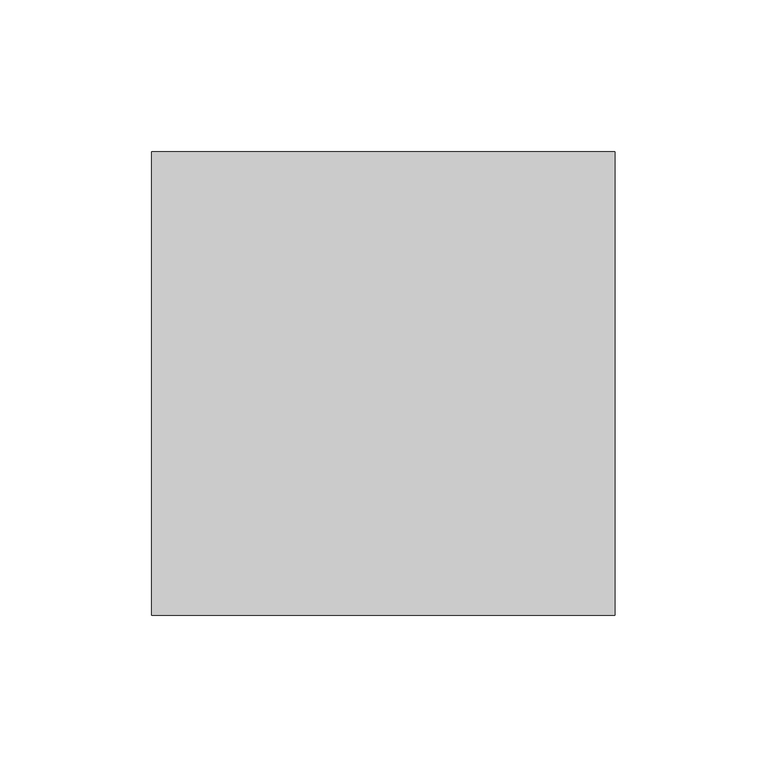
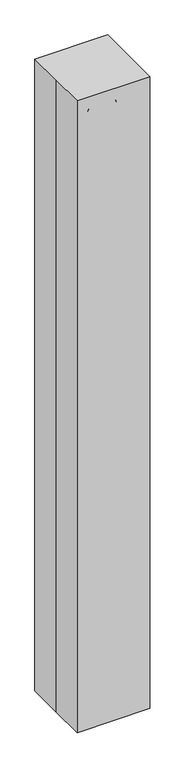
"""IFC4 building model written with IfcOpenShell, lengths in millimetres: proxy geometry, M8515 - Gastroscope, Fiberoptic, Therapeutic : M8515 - Gastroscope, Fiberoptic, Therapeutic."""

import ifcopenshell
import ifcopenshell.guid

model = None  # the IFC model being written
_history = None  # IfcOwnerHistory: only IFC2X3 demands one
_inside = {}  # id of a spatial element -> (the spatial element, [elements in it])
_under = {}  # id of a project, library or spatial element -> (it, [spatial elements below it])
_declared = {}  # id of a project -> (the project, [libraries it declares])
_typed = {}  # id of a type object -> (the type object, [elements of that type])
_made_of = {}  # id of a material, layer set ... -> (it, [elements and type objects made of it])


def new_model(schema):
    """Start an empty IFC model of exactly this schema.

    Asked for "IFC4X3", IfcOpenShell would pick the latest addendum, in which some entities
    have other attributes; the version numbers below select the first issue.
    IFC2X3 requires an IfcOwnerHistory on every rooted entity: one is made here for all.
    """
    global model, _history
    if schema == "IFC4X3":
        model = ifcopenshell.file(schema_version=(4, 3, 0, 0))
    else:
        model = ifcopenshell.file(schema=schema)
    _inside.clear()
    _under.clear()
    _declared.clear()
    _typed.clear()
    _made_of.clear()
    _history = None
    if model.schema == "IFC2X3":
        org = make("IfcOrganization", Name="unknown")
        user = make(
            "IfcPersonAndOrganization",
            ThePerson=make("IfcPerson", FamilyName="unknown"),
            TheOrganization=org,
        )
        app = make(
            "IfcApplication",
            ApplicationDeveloper=org,
            Version="unknown",
            ApplicationFullName="unknown",
            ApplicationIdentifier="unknown",
        )
        _history = make(
            "IfcOwnerHistory",
            OwningUser=user,
            OwningApplication=app,
            ChangeAction="ADDED",
            CreationDate=0,
        )
    return model


def make(cls, **values):
    """One entity of the class cls with the attributes given. An attribute that is None is left unset."""
    return model.create_entity(
        cls, **{name: value for name, value in values.items() if value is not None}
    )


def rooted(cls, **values):
    """An entity with a GlobalId (a new one), such as an element, a storey or a relation."""
    return make(cls, GlobalId=ifcopenshell.guid.new(), OwnerHistory=_history, **values)


def si_unit(unit_type, name, prefix=None):
    """IfcSIUnit, for example si_unit("LENGTHUNIT", "METRE", prefix="MILLI")."""
    return make("IfcSIUnit", UnitType=unit_type, Prefix=prefix, Name=name)


def assignment(units):
    """IfcUnitAssignment: the units of a project."""
    return None if units is None else make("IfcUnitAssignment", Units=units)


def point(xyz):
    """IfcCartesianPoint."""
    return None if xyz is None else make("IfcCartesianPoint", Coordinates=xyz)


def direction(xyz):
    """IfcDirection."""
    return None if xyz is None else make("IfcDirection", DirectionRatios=xyz)


def frame(location, z_axis=None, x_axis=None):
    """IfcAxis2Placement3D, a coordinate frame: its origin and axes. An axis left out is left unset."""
    return make(
        "IfcAxis2Placement3D",
        Location=point(location),
        Axis=direction(z_axis),
        RefDirection=direction(x_axis),
    )


def origin():
    """The frame at (0, 0, 0) with its axes left unset."""
    return frame((0.0, 0.0, 0.0))


def origin_with_axes():
    """The frame at (0, 0, 0) with the z axis (0, 0, 1) and the x axis (1, 0, 0) written out."""
    return frame((0.0, 0.0, 0.0), z_axis=(0.0, 0.0, 1.0), x_axis=(1.0, 0.0, 0.0))


def place(relative_to, where):
    """IfcLocalPlacement: puts the frame where relative to a parent placement (None: the world)."""
    return make(
        "IfcLocalPlacement", PlacementRelTo=relative_to, RelativePlacement=where
    )


def context(
    kind, dimensions, precision=None, world=None, true_north=None, identifier=None
):
    """IfcGeometricRepresentationContext, for example the 3D "Model" context."""
    return make(
        "IfcGeometricRepresentationContext",
        ContextIdentifier=identifier,
        ContextType=kind,
        CoordinateSpaceDimension=dimensions,
        Precision=precision,
        WorldCoordinateSystem=world,
        TrueNorth=true_north,
    )


def project(units=None, contexts=None):
    """IfcProject with its units and contexts."""
    return rooted(
        "IfcProject",
        Name="project",
        RepresentationContexts=contexts,
        UnitsInContext=assignment(units),
    )


def spatial(cls, under=None, at=None, **own):
    """A site, building, storey or space (cls), placed at a placement, below another one or the project."""
    s = rooted(cls, ObjectPlacement=at, **own)
    if under is not None:
        _under.setdefault(under.id(), (under, []))[1].append(s)
    return s


def polyline(points):
    """IfcPolyline through the points."""
    return make("IfcPolyline", Points=[point(p) for p in points])


def circle_curve(where, radius):
    """IfcCircle in the frame where."""
    return make("IfcCircle", Position=where, Radius=radius)


def ellipse_curve(where, semi_axis1, semi_axis2):
    """IfcEllipse in the frame where."""
    return make(
        "IfcEllipse", Position=where, SemiAxis1=semi_axis1, SemiAxis2=semi_axis2
    )


def trimmed(basis, trim1, trim2, sense, master):
    """IfcTrimmedCurve: the piece of a basis curve between two trims."""
    return make(
        "IfcTrimmedCurve",
        BasisCurve=basis,
        Trim1=trim1,
        Trim2=trim2,
        SenseAgreement=sense,
        MasterRepresentation=master,
    )


def outline(outer, holes=None, kind="AREA"):
    """IfcArbitraryClosedProfileDef: a profile drawn as a closed curve; with holes, ...WithVoids."""
    if holes is None:
        return make("IfcArbitraryClosedProfileDef", ProfileType=kind, OuterCurve=outer)
    return make(
        "IfcArbitraryProfileDefWithVoids",
        ProfileType=kind,
        OuterCurve=outer,
        InnerCurves=holes,
    )


def extrude(swept, where, along, depth):
    """IfcExtrudedAreaSolid: the profile swept, set in the frame where, extruded along a direction by depth."""
    return make(
        "IfcExtrudedAreaSolid",
        SweptArea=swept,
        Position=where,
        ExtrudedDirection=direction(along),
        Depth=depth,
    )


def shape(context_of_items, identifier, shape_type, items):
    """IfcShapeRepresentation: the items that make up one representation, for example the "Body"."""
    return make(
        "IfcShapeRepresentation",
        ContextOfItems=context_of_items,
        RepresentationIdentifier=identifier,
        RepresentationType=shape_type,
        Items=items,
    )


def source(mapping_origin, context_of_items, identifier, shape_type, items):
    """IfcRepresentationMap: a shape defined once, which mapped items show again and again."""
    return make(
        "IfcRepresentationMap",
        MappingOrigin=mapping_origin,
        MappedRepresentation=shape(context_of_items, identifier, shape_type, items),
    )


def transform(
    local_origin,
    x_axis=None,
    y_axis=None,
    z_axis=None,
    scale=None,
    scale2=None,
    scale3=None,
    uniform=True,
):
    """IfcCartesianTransformationOperator3D, or its non-uniform kind. x_axis, y_axis, z_axis: its Axis1, 2, 3."""
    if uniform:
        return make(
            "IfcCartesianTransformationOperator3D",
            Axis1=direction(x_axis),
            Axis2=direction(y_axis),
            LocalOrigin=point(local_origin),
            Scale=scale,
            Axis3=direction(z_axis),
        )
    return make(
        "IfcCartesianTransformationOperator3DnonUniform",
        Axis1=direction(x_axis),
        Axis2=direction(y_axis),
        LocalOrigin=point(local_origin),
        Scale=scale,
        Axis3=direction(z_axis),
        Scale2=scale2,
        Scale3=scale3,
    )


def mapped(mapping_source, mapping_target):
    """IfcMappedItem: shows the shape of a source again, moved by a transform."""
    return make(
        "IfcMappedItem", MappingSource=mapping_source, MappingTarget=mapping_target
    )


def made_of(thing, what):
    """Note that an element or type object is made of a material, layer set ...; save() writes the relation."""
    if what is not None:
        _made_of.setdefault(what.id(), (what, []))[1].append(thing)
    return thing


def element(
    cls,
    number,
    at=None,
    inside=None,
    cuts=None,
    type_object=None,
    material=None,
    context=None,
    identifier="Body",
    shape_type=None,
    held_by="IfcProductDefinitionShape",
    body=None,
    shapes=None,
    **own,
):
    """One element of the class cls, such as IfcWall. Its Tag is "e" and its number.

    at: its placement. inside: the storey or other place that contains it. cuts: it is an
    opening in that element (IfcRelVoidsElement). A single representation is given by context,
    identifier, shape_type and body (its items); several are given by shapes. held_by: the class
    of the entity that holds the representations. save() writes the other relations.
    """
    e = rooted(cls, Tag="e%d" % number, ObjectPlacement=at, **own)
    if body is not None:
        shapes = [shape(context, identifier, shape_type, body)]
    if shapes is not None:
        e.Representation = make(held_by, Representations=shapes)
    if inside is not None:
        _inside.setdefault(inside.id(), (inside, []))[1].append(e)
    if cuts is not None:
        rooted(
            "IfcRelVoidsElement", RelatingBuildingElement=cuts, RelatedOpeningElement=e
        )
    if type_object is not None:
        _typed.setdefault(type_object.id(), (type_object, []))[1].append(e)
    return made_of(e, material)


def aggregate(whole, parts):
    """IfcRelAggregates: a whole, such as a stair, and the parts it consists of."""
    return rooted("IfcRelAggregates", RelatingObject=whole, RelatedObjects=parts)


def save(model, path):
    """Write the relations noted so far, then the file.

    IfcRelAggregates (storeys below a building ...), IfcRelContainedInSpatialStructure (elements
    in a storey), IfcRelDefinesByType, IfcRelAssociatesMaterial and IfcRelDeclares: one each for
    every whole, place, type object, material and project.
    """
    for whole, parts in _under.values():
        aggregate(whole, parts)
    for where, things in _inside.values():
        rooted(
            "IfcRelContainedInSpatialStructure",
            RelatedElements=things,
            RelatingStructure=where,
        )
    for kind, things in _typed.values():
        rooted("IfcRelDefinesByType", RelatedObjects=things, RelatingType=kind)
    for what, things in _made_of.values():
        rooted("IfcRelAssociatesMaterial", RelatedObjects=things, RelatingMaterial=what)
    for by, libraries in _declared.values():
        rooted("IfcRelDeclares", RelatingContext=by, RelatedDefinitions=libraries)
    model.write(path)


def plane_surface(at):
    """IfcPlane: the flat surface through the origin of the frame at, square to its z axis."""
    return make("IfcPlane", Position=at)


def cylinder_surface(at, radius):
    """IfcCylindricalSurface: all points at the distance radius from the z axis of the frame at."""
    return make("IfcCylindricalSurface", Position=at, Radius=radius)


def revolved_surface(curve, axis_point, axis_direction):
    """IfcSurfaceOfRevolution: the curve turned about the line through axis_point along axis_direction."""
    return make(
        "IfcSurfaceOfRevolution",
        SweptCurve=make("IfcArbitraryOpenProfileDef", ProfileType="CURVE", Curve=curve),
        AxisPosition=make("IfcAxis1Placement", Location=point(axis_point), Axis=direction(axis_direction)),
    )


def advanced_brep(points, edges, surfaces, faces):
    """IfcAdvancedBrep: a solid bounded by faces that lie on surfaces and meet in shared edges.

    An edge is (start, end): straight between two places in points (the first is 0);
    or (start, end, curve); or (start, end, curve, False) where it runs against its curve.
    A face is (place in surfaces, loops), or (place, loops, False) where it looks against
    its surface's normal. A loop lists edges by number (the first is 1), with a minus sign
    where the edge is run from its end to its start. The first loop is the outer one.
    """
    corners = [point(p) for p in points]
    vertices = [make("IfcVertexPoint", VertexGeometry=c) for c in corners]
    made = []
    for start, end, *more in edges:
        made.append(
            make(
                "IfcEdgeCurve",
                EdgeStart=vertices[start],
                EdgeEnd=vertices[end],
                EdgeGeometry=more[0] if more else make("IfcPolyline", Points=[corners[start], corners[end]]),
                SameSense=more[1] if len(more) > 1 else True,
            )
        )
    hull = []
    for where, loops, *sense in faces:
        bounds = []
        for j, loop in enumerate(loops):
            ring = [make("IfcOrientedEdge", EdgeElement=made[abs(k) - 1], Orientation=k > 0) for k in loop]
            bounds.append(
                make(
                    "IfcFaceOuterBound" if j == 0 else "IfcFaceBound",
                    Bound=make("IfcEdgeLoop", EdgeList=ring),
                    Orientation=True,
                )
            )
        hull.append(make("IfcAdvancedFace", Bounds=bounds, FaceSurface=surfaces[where], SameSense=sense[0] if sense else True))
    return make("IfcAdvancedBrep", Outer=make("IfcClosedShell", CfsFaces=hull))


def specialty_equipment_7175bac1(model_context):
    return source(origin(), model_context, "Body", "SolidModel", [
        extrude(outline(polyline([(-12.7, -34.925), (-50.8, -34.925), (-50.8, -9.525), (-12.7, -9.525), (-12.7, -34.925)])), origin_with_axes(), (0.0, 0.0, 1.0), 101.6),
        advanced_brep(
        [(-25.4, -22.225, 101.6), (-38.1, -22.225, 101.6), (25.4, -22.225, 0.0), (38.1, -22.225, 0.0), (-25.4, -22.225, 1314.45), (-38.1, -22.225, 1314.45), (38.1, -22.225, 1314.45), (25.4, -22.225, 1314.45)],
        [
            (0, 1, circle_curve(frame((-31.75, -22.225, 101.6), z_axis=(0.0, 0.0, -1.0), x_axis=(-1.0, 0.0, 0.0)), 6.35)),
            (1, 0, circle_curve(frame((-31.75, -22.225, 101.6), z_axis=(0.0, 0.0, -1.0), x_axis=(-1.0, 0.0, 0.0)), 6.35)),
            (2, 3, circle_curve(frame((31.75, -22.225, 0.0), z_axis=(0.0, 0.0, -1.0), x_axis=(1.0, 0.0, 0.0)), 6.35)),
            (3, 2, circle_curve(frame((31.75, -22.225, 0.0), z_axis=(0.0, 0.0, -1.0), x_axis=(1.0, 0.0, 0.0)), 6.35)),
            (0, 4),
            (4, 5, circle_curve(frame((-31.75, -22.225, 1314.45), z_axis=(0.0, 0.0, -1.0), x_axis=(-1.0, 0.0, 0.0)), 6.35)),
            (5, 1),
            (5, 4, circle_curve(frame((-31.75, -22.225, 1314.45), z_axis=(0.0, 0.0, -1.0), x_axis=(-1.0, 0.0, 0.0)), 6.35)),
            (6, 7, circle_curve(frame((31.75, -22.225, 1314.45), z_axis=(0.0, 0.0, -1.0), x_axis=(1.0, 0.0, 0.0)), 6.35)),
            (7, 2),
            (3, 6),
            (7, 6, circle_curve(frame((31.75, -22.225, 1314.45), z_axis=(0.0, 0.0, -1.0), x_axis=(1.0, 0.0, 0.0)), 6.35)),
            (6, 5, circle_curve(frame((0.0, -22.225, 1314.45), z_axis=(0.0, -1.0, 0.0), x_axis=(-1.0, 0.0, 0.0)), 38.1)),
            (4, 7, circle_curve(frame((0.0, -22.225, 1314.45), z_axis=(0.0, 1.0, 0.0), x_axis=(-1.0, 0.0, 0.0)), 25.4)),
        ],
        [
            plane_surface(frame((-31.75, 41.275, 101.6), z_axis=(0.0, 0.0, -1.0), x_axis=(0.0, -1.0, 0.0))),
            plane_surface(frame((31.75, 41.275, 0.0), z_axis=(0.0, 0.0, -1.0), x_axis=(0.0, -1.0, 0.0))),
            cylinder_surface(frame((-31.75, -22.225, 101.6), z_axis=(0.0, 0.0, -1.0), x_axis=(-1.0, 0.0, 0.0)), 6.35),
            cylinder_surface(frame((31.75, -22.225, 1314.45), z_axis=(0.0, 0.0, 1.0), x_axis=(1.0, 0.0, 0.0)), 6.35),
            revolved_surface(trimmed(ellipse_curve(frame((-31.75, -22.225, 1314.45), z_axis=(0.0, 0.0, -1.0), x_axis=(-1.0, 0.0, 0.0)), 6.35, 6.35), [point((-25.4, -22.225, 1314.45))], [point((-38.1, -22.225, 1314.45))], True, "CARTESIAN"), (0.0, 41.275, 1314.45), (0.0, 1.0, 0.0)),
            revolved_surface(trimmed(ellipse_curve(frame((-31.75, -22.225, 1314.45), z_axis=(0.0, 0.0, -1.0), x_axis=(-1.0, 0.0, 0.0)), 6.35, 6.35), [point((-38.1, -22.225, 1314.45))], [point((-25.4, -22.225, 1314.45))], True, "CARTESIAN"), (0.0, 41.275, 1314.45), (0.0, 1.0, 0.0)),
        ],
        [
            (0, [[1, 2]]),
            (1, [[3, 4]]),
            (2, [[-1, 5, 6, 7]]),
            (2, [[-2, -7, 8, -5]]),
            (3, [[9, 10, -4, 11]]),
            (3, [[12, -11, -3, -10]]),
            (4, [[13, -6, 14, -9]]),
            (5, [[-14, -8, -13, -12]]),
        ],
    ),
        extrude(outline(polyline([(-76.2, 76.2), (76.2, 76.2), (76.2, -76.2), (-76.2, -76.2), (-76.2, 0.0), (-76.2, 76.2)])), origin_with_axes(), (0.0, 0.0, 1.0), 1397.0),
    ])


if __name__ == "__main__":
    model = new_model("IFC4")
    model_context = context("Model", 3, world=origin())
    ifc_project = project(units=[si_unit("LENGTHUNIT", "METRE", prefix="MILLI")], contexts=[model_context])
    site = spatial("IfcSite", under=ifc_project)
    building = spatial("IfcBuilding", under=site)
    placement = place(None, origin())
    specialty_equipment_shape = specialty_equipment_7175bac1(model_context)
    element("IfcBuildingElementProxy", 1, Name="M8515 - Gastroscope, Fiberoptic, Therapeutic : M8515 - Gastroscope, Fiberoptic, Therapeutic", ObjectType="M8515 - Gastroscope, Fiberoptic, Therapeutic : M8515 - Gastroscope, Fiberoptic, Therapeutic", at=placement, inside=building, context=model_context, shape_type="MappedRepresentation", body=[
        mapped(specialty_equipment_shape, transform((0.0, 0.0, 0.0), x_axis=(1.0, 0.0, 0.0), y_axis=(0.0, 1.0, 0.0), z_axis=(0.0, 0.0, 1.0))),
    ])
    save(model, "model.ifc")

# Revit data of these elements
# Type "M8515 - Gastroscope, Fiberoptic, Therapeutic : M8515 - Gastroscope, Fiberoptic, Therapeutic"
#   Watts2 = "0"
#   Watts1 = "0"
#   Unit_Issue = "EA"
#   UTIL_6_Misc = "-"
#   UTIL_5_NonMedGas = "-"
#   UTIL_4_MiscGas = "-"
#   UTIL_3_MedGas = "-"
#   UTIL_2_Elec = "-"
#   UTIL_1_WaterDrain = "-"
#   Nomenclature = "Gastroscope, Fiberoptic, Therapeutic"
#   NSN = "6515"
#   Location [instance default] = ""
#   JSN = "M8515"
#   Fund_Source_VA = "-"
#   Fund_Source_Navy = "-"
#   Fund_Source_Army = "-"
#   Fund_Source_AF = "-"
#   ELEC_Volts2 = "0"
#   ELEC_Volts1 = "0"
#   ELEC_Phase2 = "0"
#   ELEC_Phase1 = "0"
#   ELEC_HertzSwitch = "0"
#   ELEC_HertzDependent = "0"
#   ELEC_Hertz = "0"
#   ELEC_Amps2 = "0"
#   ELEC_Amps1 = "0"
#   DetailDescription = "Flexible fiberoptic gastroscope. This scope is designed for gastrointestinal exploration, cleaning, biopsy, tissue removal and suctioning. Unit consists of a thin flexible casing with a suction adapter, an instrument channel, light guides, an objective lens with an optical image fiber cluster, an air/water channel, an eyepiece and a cable for connection to a light source. Casings and instrument channels can have varying dimensions based on gastroscope design and intended procedure. Some scopes feature dual instrument channels for more complex procedures."
#   CAT_VA = "C"
#   CAT_Navy = "C"
#   CAT_IHS = "-"
#   CAT_Army = "C"
#   CAT_AF = "C"
#   BTUperhour = "0"
#   Weight_IP = 10
#   DIM_Width_IP = 0' - 6"
#   DIM_Height_IP = 0' - 6"
#   DIM_Depth_IP = 4' - 7"
# Element 1 (IfcBuildingElementProxy, "M8515 - Gastroscope, Fiberoptic, Therapeutic : M8515 - Gastroscope, Fiberoptic, Therapeutic")
#   Location = "TREE1"
#   Materials on its faces: "EquipSpace"
# Materials
#   "EquipSpace": class "Miscellaneous", colour RGB 221 217 195, transparency 0.5
